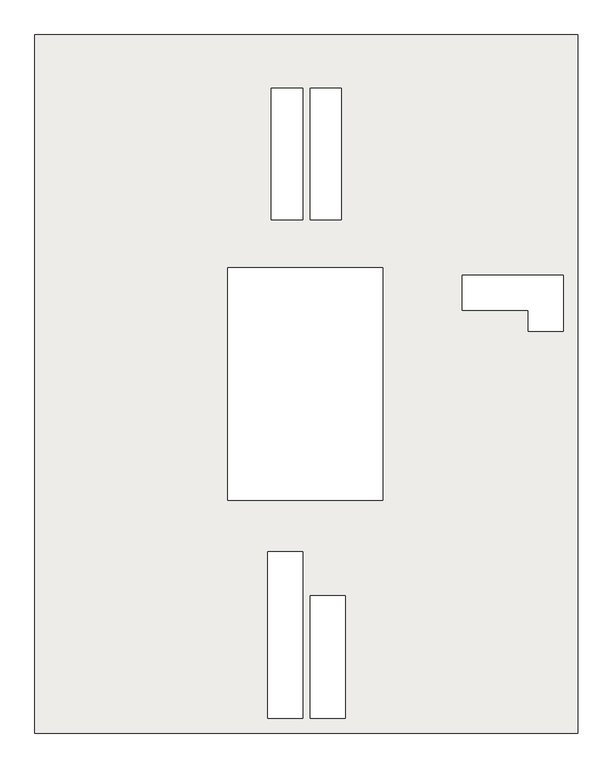
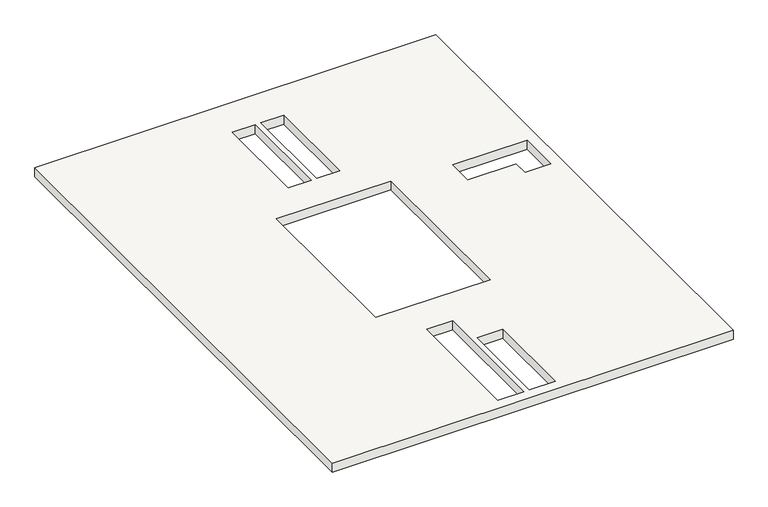
"""IFC4 building model written with IfcOpenShell, lengths in millimetres: slab geometry, Holzdecke 142136 : Holzdecke 142136."""

import ifcopenshell
import ifcopenshell.guid

model = None  # the IFC model being written
_history = None  # IfcOwnerHistory: only IFC2X3 demands one
_inside = {}  # id of a spatial element -> (the spatial element, [elements in it])
_under = {}  # id of a project, library or spatial element -> (it, [spatial elements below it])
_declared = {}  # id of a project -> (the project, [libraries it declares])
_typed = {}  # id of a type object -> (the type object, [elements of that type])
_made_of = {}  # id of a material, layer set ... -> (it, [elements and type objects made of it])


def new_model(schema):
    """Start an empty IFC model of exactly this schema.

    Asked for "IFC4X3", IfcOpenShell would pick the latest addendum, in which some entities
    have other attributes; the version numbers below select the first issue.
    IFC2X3 requires an IfcOwnerHistory on every rooted entity: one is made here for all.
    """
    global model, _history
    if schema == "IFC4X3":
        model = ifcopenshell.file(schema_version=(4, 3, 0, 0))
    else:
        model = ifcopenshell.file(schema=schema)
    _inside.clear()
    _under.clear()
    _declared.clear()
    _typed.clear()
    _made_of.clear()
    _history = None
    if model.schema == "IFC2X3":
        org = make("IfcOrganization", Name="unknown")
        user = make(
            "IfcPersonAndOrganization",
            ThePerson=make("IfcPerson", FamilyName="unknown"),
            TheOrganization=org,
        )
        app = make(
            "IfcApplication",
            ApplicationDeveloper=org,
            Version="unknown",
            ApplicationFullName="unknown",
            ApplicationIdentifier="unknown",
        )
        _history = make(
            "IfcOwnerHistory",
            OwningUser=user,
            OwningApplication=app,
            ChangeAction="ADDED",
            CreationDate=0,
        )
    return model


def make(cls, **values):
    """One entity of the class cls with the attributes given. An attribute that is None is left unset."""
    return model.create_entity(
        cls, **{name: value for name, value in values.items() if value is not None}
    )


def rooted(cls, **values):
    """An entity with a GlobalId (a new one), such as an element, a storey or a relation."""
    return make(cls, GlobalId=ifcopenshell.guid.new(), OwnerHistory=_history, **values)


def si_unit(unit_type, name, prefix=None):
    """IfcSIUnit, for example si_unit("LENGTHUNIT", "METRE", prefix="MILLI")."""
    return make("IfcSIUnit", UnitType=unit_type, Prefix=prefix, Name=name)


def assignment(units):
    """IfcUnitAssignment: the units of a project."""
    return None if units is None else make("IfcUnitAssignment", Units=units)


def point(xyz):
    """IfcCartesianPoint."""
    return None if xyz is None else make("IfcCartesianPoint", Coordinates=xyz)


def direction(xyz):
    """IfcDirection."""
    return None if xyz is None else make("IfcDirection", DirectionRatios=xyz)


def frame(location, z_axis=None, x_axis=None):
    """IfcAxis2Placement3D, a coordinate frame: its origin and axes. An axis left out is left unset."""
    return make(
        "IfcAxis2Placement3D",
        Location=point(location),
        Axis=direction(z_axis),
        RefDirection=direction(x_axis),
    )


def origin():
    """The frame at (0, 0, 0) with its axes left unset."""
    return frame((0.0, 0.0, 0.0))


def place(relative_to, where):
    """IfcLocalPlacement: puts the frame where relative to a parent placement (None: the world)."""
    return make(
        "IfcLocalPlacement", PlacementRelTo=relative_to, RelativePlacement=where
    )


def context(
    kind, dimensions, precision=None, world=None, true_north=None, identifier=None
):
    """IfcGeometricRepresentationContext, for example the 3D "Model" context."""
    return make(
        "IfcGeometricRepresentationContext",
        ContextIdentifier=identifier,
        ContextType=kind,
        CoordinateSpaceDimension=dimensions,
        Precision=precision,
        WorldCoordinateSystem=world,
        TrueNorth=true_north,
    )


def project(units=None, contexts=None):
    """IfcProject with its units and contexts."""
    return rooted(
        "IfcProject",
        Name="project",
        RepresentationContexts=contexts,
        UnitsInContext=assignment(units),
    )


def spatial(cls, under=None, at=None, **own):
    """A site, building, storey or space (cls), placed at a placement, below another one or the project."""
    s = rooted(cls, ObjectPlacement=at, **own)
    if under is not None:
        _under.setdefault(under.id(), (under, []))[1].append(s)
    return s


def polyline(points):
    """IfcPolyline through the points."""
    return make("IfcPolyline", Points=[point(p) for p in points])


def outline(outer, holes=None, kind="AREA"):
    """IfcArbitraryClosedProfileDef: a profile drawn as a closed curve; with holes, ...WithVoids."""
    if holes is None:
        return make("IfcArbitraryClosedProfileDef", ProfileType=kind, OuterCurve=outer)
    return make(
        "IfcArbitraryProfileDefWithVoids",
        ProfileType=kind,
        OuterCurve=outer,
        InnerCurves=holes,
    )


def extrude(swept, where, along, depth):
    """IfcExtrudedAreaSolid: the profile swept, set in the frame where, extruded along a direction by depth."""
    return make(
        "IfcExtrudedAreaSolid",
        SweptArea=swept,
        Position=where,
        ExtrudedDirection=direction(along),
        Depth=depth,
    )


def shape(context_of_items, identifier, shape_type, items):
    """IfcShapeRepresentation: the items that make up one representation, for example the "Body"."""
    return make(
        "IfcShapeRepresentation",
        ContextOfItems=context_of_items,
        RepresentationIdentifier=identifier,
        RepresentationType=shape_type,
        Items=items,
    )


def source(mapping_origin, context_of_items, identifier, shape_type, items):
    """IfcRepresentationMap: a shape defined once, which mapped items show again and again."""
    return make(
        "IfcRepresentationMap",
        MappingOrigin=mapping_origin,
        MappedRepresentation=shape(context_of_items, identifier, shape_type, items),
    )


def transform(
    local_origin,
    x_axis=None,
    y_axis=None,
    z_axis=None,
    scale=None,
    scale2=None,
    scale3=None,
    uniform=True,
):
    """IfcCartesianTransformationOperator3D, or its non-uniform kind. x_axis, y_axis, z_axis: its Axis1, 2, 3."""
    if uniform:
        return make(
            "IfcCartesianTransformationOperator3D",
            Axis1=direction(x_axis),
            Axis2=direction(y_axis),
            LocalOrigin=point(local_origin),
            Scale=scale,
            Axis3=direction(z_axis),
        )
    return make(
        "IfcCartesianTransformationOperator3DnonUniform",
        Axis1=direction(x_axis),
        Axis2=direction(y_axis),
        LocalOrigin=point(local_origin),
        Scale=scale,
        Axis3=direction(z_axis),
        Scale2=scale2,
        Scale3=scale3,
    )


def mapped(mapping_source, mapping_target):
    """IfcMappedItem: shows the shape of a source again, moved by a transform."""
    return make(
        "IfcMappedItem", MappingSource=mapping_source, MappingTarget=mapping_target
    )


def made_of(thing, what):
    """Note that an element or type object is made of a material, layer set ...; save() writes the relation."""
    if what is not None:
        _made_of.setdefault(what.id(), (what, []))[1].append(thing)
    return thing


def element(
    cls,
    number,
    at=None,
    inside=None,
    cuts=None,
    type_object=None,
    material=None,
    context=None,
    identifier="Body",
    shape_type=None,
    held_by="IfcProductDefinitionShape",
    body=None,
    shapes=None,
    **own,
):
    """One element of the class cls, such as IfcWall. Its Tag is "e" and its number.

    at: its placement. inside: the storey or other place that contains it. cuts: it is an
    opening in that element (IfcRelVoidsElement). A single representation is given by context,
    identifier, shape_type and body (its items); several are given by shapes. held_by: the class
    of the entity that holds the representations. save() writes the other relations.
    """
    e = rooted(cls, Tag="e%d" % number, ObjectPlacement=at, **own)
    if body is not None:
        shapes = [shape(context, identifier, shape_type, body)]
    if shapes is not None:
        e.Representation = make(held_by, Representations=shapes)
    if inside is not None:
        _inside.setdefault(inside.id(), (inside, []))[1].append(e)
    if cuts is not None:
        rooted(
            "IfcRelVoidsElement", RelatingBuildingElement=cuts, RelatedOpeningElement=e
        )
    if type_object is not None:
        _typed.setdefault(type_object.id(), (type_object, []))[1].append(e)
    return made_of(e, material)


def aggregate(whole, parts):
    """IfcRelAggregates: a whole, such as a stair, and the parts it consists of."""
    return rooted("IfcRelAggregates", RelatingObject=whole, RelatedObjects=parts)


def save(model, path):
    """Write the relations noted so far, then the file.

    IfcRelAggregates (storeys below a building ...), IfcRelContainedInSpatialStructure (elements
    in a storey), IfcRelDefinesByType, IfcRelAssociatesMaterial and IfcRelDeclares: one each for
    every whole, place, type object, material and project.
    """
    for whole, parts in _under.values():
        aggregate(whole, parts)
    for where, things in _inside.values():
        rooted(
            "IfcRelContainedInSpatialStructure",
            RelatedElements=things,
            RelatingStructure=where,
        )
    for kind, things in _typed.values():
        rooted("IfcRelDefinesByType", RelatedObjects=things, RelatingType=kind)
    for what, things in _made_of.values():
        rooted("IfcRelAssociatesMaterial", RelatedObjects=things, RelatingMaterial=what)
    for by, libraries in _declared.values():
        rooted("IfcRelDeclares", RelatingContext=by, RelatedDefinitions=libraries)
    model.write(path)


def slab_52cff1b9(model_context):
    return source(origin(), model_context, "Body", "SweptSolid", [
        extrude(outline(polyline([(172797.7593015, 28481.9343946), (158797.7593015, 28481.9343946), (158797.7593015, 46484.7962965), (172797.7593015, 46484.7962965), (172797.7593015, 28481.9343946)]), holes=[polyline([(167772.7593015, 40484.7962965), (163772.7593015, 40484.7962965), (163772.7593015, 34484.7962965), (167772.7593015, 34484.7962965), (167772.7593015, 40484.7962965)]), polyline([(165697.7593015, 33159.7962965), (164797.7593015, 33159.7962965), (164797.7593015, 28861.9343946), (165697.7593015, 28861.9343946), (165697.7593015, 33159.7962965)]), polyline([(165897.7593015, 32021.9343946), (165897.7593015, 29779.7962965), (165897.7593015, 28861.9343946), (166797.7593015, 28861.9343946), (166797.7593015, 32021.9343946), (165897.7593015, 32021.9343946)]), polyline([(171517.7593015, 38844.7962965), (172417.7593015, 38844.7962965), (172417.7593015, 40284.7962965), (169822.7593015, 40284.7962965), (169822.7593015, 39384.7962965), (171517.7593015, 39384.7962965), (171517.7593015, 38844.7962965)]), polyline([(165897.7593015, 45104.7962965), (165897.7593015, 41724.7962965), (166697.7593015, 41724.7962965), (166697.7593015, 45104.7962965), (165897.7593015, 45104.7962965)]), polyline([(164897.7593015, 41724.7962965), (165697.7593015, 41724.7962965), (165697.7593015, 45104.7962965), (164897.7593015, 45104.7962965), (164897.7593015, 41724.7962965)])]), frame((0.0, 0.0, 5830.0), z_axis=(0.0, 0.0, 1.0), x_axis=(1.0, 0.0, 0.0)), (0.0, 0.0, 1.0), 330.0),
    ])


if __name__ == "__main__":
    model = new_model("IFC4")
    model_context = context("Model", 3, world=origin())
    ifc_project = project(units=[si_unit("LENGTHUNIT", "METRE", prefix="MILLI")], contexts=[model_context])
    site = spatial("IfcSite", under=ifc_project)
    building = spatial("IfcBuilding", under=site)
    placement = place(None, origin())
    slab_shape = slab_52cff1b9(model_context)
    element("IfcSlab", 1, ObjectType="Holzdecke 142136 : Holzdecke 142136", at=placement, inside=building, context=model_context, shape_type="MappedRepresentation", body=[
        mapped(slab_shape, transform((0.0, 0.0, 0.0), x_axis=(1.0, 0.0, 0.0), y_axis=(0.0, 1.0, 0.0), z_axis=(0.0, 0.0, 1.0))),
    ])
    save(model, "model.ifc")

# Revit data of these elements
# Type "Holzdecke 142136 : Holzdecke 142136"
#   Abrechnungsart = "m²"
#   Allright_Bauteil_ID = "0123De 0783954319"
#   Bezeichnung = "Holzdecke"
#   Codetext = "D-HOLZBALKEN1\\"
#   Gewerk = "Zimmer- und Holzbauarbeiten"
#   Material = "Holz"
#   Objektname = "Brettstapeldecke"
#   NameOverride = "Holzdecke"
#   Reference = "Holzdecke"
#   Status = "NEW"
#   PitchAngle = 0.00°
#   ThermalTransmittance = 0.0000 BTU/(h·ft²·°F)
#   2D Interaktion = yes
#   Combustible = no
#   Compartmentation = no
#   IsExternal = no
#   LoadBearing = yes
# Element 1 (IfcSlab, "Holzdecke 142136 : Holzdecke 142136")
#   Materials on its faces: "holzschalung"
# Materials
#   "holzschalung": class "Unassigned", colour RGB 128 128 128, transparency 0
